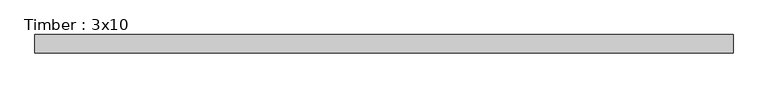
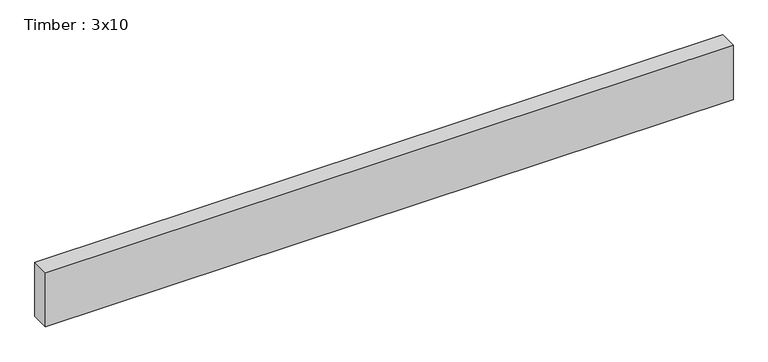
"""IFC4 building model written with IfcOpenShell, lengths in millimetres: beam geometry, Timber : 3x10."""

import ifcopenshell
import ifcopenshell.guid

model = None  # the IFC model being written
_history = None  # IfcOwnerHistory: only IFC2X3 demands one
_inside = {}  # id of a spatial element -> (the spatial element, [elements in it])
_under = {}  # id of a project, library or spatial element -> (it, [spatial elements below it])
_declared = {}  # id of a project -> (the project, [libraries it declares])
_typed = {}  # id of a type object -> (the type object, [elements of that type])
_made_of = {}  # id of a material, layer set ... -> (it, [elements and type objects made of it])


def new_model(schema):
    """Start an empty IFC model of exactly this schema.

    Asked for "IFC4X3", IfcOpenShell would pick the latest addendum, in which some entities
    have other attributes; the version numbers below select the first issue.
    IFC2X3 requires an IfcOwnerHistory on every rooted entity: one is made here for all.
    """
    global model, _history
    if schema == "IFC4X3":
        model = ifcopenshell.file(schema_version=(4, 3, 0, 0))
    else:
        model = ifcopenshell.file(schema=schema)
    _inside.clear()
    _under.clear()
    _declared.clear()
    _typed.clear()
    _made_of.clear()
    _history = None
    if model.schema == "IFC2X3":
        org = make("IfcOrganization", Name="unknown")
        user = make(
            "IfcPersonAndOrganization",
            ThePerson=make("IfcPerson", FamilyName="unknown"),
            TheOrganization=org,
        )
        app = make(
            "IfcApplication",
            ApplicationDeveloper=org,
            Version="unknown",
            ApplicationFullName="unknown",
            ApplicationIdentifier="unknown",
        )
        _history = make(
            "IfcOwnerHistory",
            OwningUser=user,
            OwningApplication=app,
            ChangeAction="ADDED",
            CreationDate=0,
        )
    return model


def make(cls, **values):
    """One entity of the class cls with the attributes given. An attribute that is None is left unset."""
    return model.create_entity(
        cls, **{name: value for name, value in values.items() if value is not None}
    )


def rooted(cls, **values):
    """An entity with a GlobalId (a new one), such as an element, a storey or a relation."""
    return make(cls, GlobalId=ifcopenshell.guid.new(), OwnerHistory=_history, **values)


def si_unit(unit_type, name, prefix=None):
    """IfcSIUnit, for example si_unit("LENGTHUNIT", "METRE", prefix="MILLI")."""
    return make("IfcSIUnit", UnitType=unit_type, Prefix=prefix, Name=name)


def assignment(units):
    """IfcUnitAssignment: the units of a project."""
    return None if units is None else make("IfcUnitAssignment", Units=units)


def point(xyz):
    """IfcCartesianPoint."""
    return None if xyz is None else make("IfcCartesianPoint", Coordinates=xyz)


def direction(xyz):
    """IfcDirection."""
    return None if xyz is None else make("IfcDirection", DirectionRatios=xyz)


def frame(location, z_axis=None, x_axis=None):
    """IfcAxis2Placement3D, a coordinate frame: its origin and axes. An axis left out is left unset."""
    return make(
        "IfcAxis2Placement3D",
        Location=point(location),
        Axis=direction(z_axis),
        RefDirection=direction(x_axis),
    )


def origin():
    """The frame at (0, 0, 0) with its axes left unset."""
    return frame((0.0, 0.0, 0.0))


def place(relative_to, where):
    """IfcLocalPlacement: puts the frame where relative to a parent placement (None: the world)."""
    return make(
        "IfcLocalPlacement", PlacementRelTo=relative_to, RelativePlacement=where
    )


def context(
    kind, dimensions, precision=None, world=None, true_north=None, identifier=None
):
    """IfcGeometricRepresentationContext, for example the 3D "Model" context."""
    return make(
        "IfcGeometricRepresentationContext",
        ContextIdentifier=identifier,
        ContextType=kind,
        CoordinateSpaceDimension=dimensions,
        Precision=precision,
        WorldCoordinateSystem=world,
        TrueNorth=true_north,
    )


def project(units=None, contexts=None):
    """IfcProject with its units and contexts."""
    return rooted(
        "IfcProject",
        Name="project",
        RepresentationContexts=contexts,
        UnitsInContext=assignment(units),
    )


def spatial(cls, under=None, at=None, **own):
    """A site, building, storey or space (cls), placed at a placement, below another one or the project."""
    s = rooted(cls, ObjectPlacement=at, **own)
    if under is not None:
        _under.setdefault(under.id(), (under, []))[1].append(s)
    return s


def polyline(points):
    """IfcPolyline through the points."""
    return make("IfcPolyline", Points=[point(p) for p in points])


def outline(outer, holes=None, kind="AREA"):
    """IfcArbitraryClosedProfileDef: a profile drawn as a closed curve; with holes, ...WithVoids."""
    if holes is None:
        return make("IfcArbitraryClosedProfileDef", ProfileType=kind, OuterCurve=outer)
    return make(
        "IfcArbitraryProfileDefWithVoids",
        ProfileType=kind,
        OuterCurve=outer,
        InnerCurves=holes,
    )


def extrude(swept, where, along, depth):
    """IfcExtrudedAreaSolid: the profile swept, set in the frame where, extruded along a direction by depth."""
    return make(
        "IfcExtrudedAreaSolid",
        SweptArea=swept,
        Position=where,
        ExtrudedDirection=direction(along),
        Depth=depth,
    )


def shape(context_of_items, identifier, shape_type, items):
    """IfcShapeRepresentation: the items that make up one representation, for example the "Body"."""
    return make(
        "IfcShapeRepresentation",
        ContextOfItems=context_of_items,
        RepresentationIdentifier=identifier,
        RepresentationType=shape_type,
        Items=items,
    )


def source(mapping_origin, context_of_items, identifier, shape_type, items):
    """IfcRepresentationMap: a shape defined once, which mapped items show again and again."""
    return make(
        "IfcRepresentationMap",
        MappingOrigin=mapping_origin,
        MappedRepresentation=shape(context_of_items, identifier, shape_type, items),
    )


def transform(
    local_origin,
    x_axis=None,
    y_axis=None,
    z_axis=None,
    scale=None,
    scale2=None,
    scale3=None,
    uniform=True,
):
    """IfcCartesianTransformationOperator3D, or its non-uniform kind. x_axis, y_axis, z_axis: its Axis1, 2, 3."""
    if uniform:
        return make(
            "IfcCartesianTransformationOperator3D",
            Axis1=direction(x_axis),
            Axis2=direction(y_axis),
            LocalOrigin=point(local_origin),
            Scale=scale,
            Axis3=direction(z_axis),
        )
    return make(
        "IfcCartesianTransformationOperator3DnonUniform",
        Axis1=direction(x_axis),
        Axis2=direction(y_axis),
        LocalOrigin=point(local_origin),
        Scale=scale,
        Axis3=direction(z_axis),
        Scale2=scale2,
        Scale3=scale3,
    )


def mapped(mapping_source, mapping_target):
    """IfcMappedItem: shows the shape of a source again, moved by a transform."""
    return make(
        "IfcMappedItem", MappingSource=mapping_source, MappingTarget=mapping_target
    )


def made_of(thing, what):
    """Note that an element or type object is made of a material, layer set ...; save() writes the relation."""
    if what is not None:
        _made_of.setdefault(what.id(), (what, []))[1].append(thing)
    return thing


def element(
    cls,
    number,
    at=None,
    inside=None,
    cuts=None,
    type_object=None,
    material=None,
    context=None,
    identifier="Body",
    shape_type=None,
    held_by="IfcProductDefinitionShape",
    body=None,
    shapes=None,
    **own,
):
    """One element of the class cls, such as IfcWall. Its Tag is "e" and its number.

    at: its placement. inside: the storey or other place that contains it. cuts: it is an
    opening in that element (IfcRelVoidsElement). A single representation is given by context,
    identifier, shape_type and body (its items); several are given by shapes. held_by: the class
    of the entity that holds the representations. save() writes the other relations.
    """
    e = rooted(cls, Tag="e%d" % number, ObjectPlacement=at, **own)
    if body is not None:
        shapes = [shape(context, identifier, shape_type, body)]
    if shapes is not None:
        e.Representation = make(held_by, Representations=shapes)
    if inside is not None:
        _inside.setdefault(inside.id(), (inside, []))[1].append(e)
    if cuts is not None:
        rooted(
            "IfcRelVoidsElement", RelatingBuildingElement=cuts, RelatedOpeningElement=e
        )
    if type_object is not None:
        _typed.setdefault(type_object.id(), (type_object, []))[1].append(e)
    return made_of(e, material)


def aggregate(whole, parts):
    """IfcRelAggregates: a whole, such as a stair, and the parts it consists of."""
    return rooted("IfcRelAggregates", RelatingObject=whole, RelatedObjects=parts)


def save(model, path):
    """Write the relations noted so far, then the file.

    IfcRelAggregates (storeys below a building ...), IfcRelContainedInSpatialStructure (elements
    in a storey), IfcRelDefinesByType, IfcRelAssociatesMaterial and IfcRelDeclares: one each for
    every whole, place, type object, material and project.
    """
    for whole, parts in _under.values():
        aggregate(whole, parts)
    for where, things in _inside.values():
        rooted(
            "IfcRelContainedInSpatialStructure",
            RelatedElements=things,
            RelatingStructure=where,
        )
    for kind, things in _typed.values():
        rooted("IfcRelDefinesByType", RelatedObjects=things, RelatingType=kind)
    for what, things in _made_of.values():
        rooted("IfcRelAssociatesMaterial", RelatedObjects=things, RelatingMaterial=what)
    for by, libraries in _declared.values():
        rooted("IfcRelDeclares", RelatingContext=by, RelatedDefinitions=libraries)
    model.write(path)


def timber_3x10_f201f224(model_context):
    return source(origin(), model_context, "Body", "SweptSolid", [
        extrude(outline(polyline([(1446.1657684, 38.1), (1446.1657684, -38.1), (-1446.1657684, -38.1), (-1446.1657684, 38.1), (1446.1657684, 38.1)])), frame((0.0, 0.0, -120.65), z_axis=(0.0, 0.0, 1.0), x_axis=(1.0, 0.0, 0.0)), (0.0, 0.0, 1.0), 241.3),
    ])


if __name__ == "__main__":
    model = new_model("IFC4")
    model_context = context("Model", 3, world=origin())
    ifc_project = project(units=[si_unit("LENGTHUNIT", "METRE", prefix="MILLI")], contexts=[model_context])
    site = spatial("IfcSite", under=ifc_project)
    building = spatial("IfcBuilding", under=site)
    placement = place(None, origin())
    timber_3x10_shape = timber_3x10_f201f224(model_context)
    element("IfcBeam", 1, ObjectType="Timber : 3x10", at=placement, inside=building, context=model_context, shape_type="MappedRepresentation", body=[
        mapped(timber_3x10_shape, transform((0.0, 0.0, 0.0), x_axis=(1.0, 0.0, 0.0), y_axis=(0.0, 1.0, 0.0), z_axis=(0.0, 0.0, 1.0))),
    ])
    save(model, "model.ifc")

# Revit data of these elements
# Type "Timber : 3x10"
#   Assembly Code = "B10"
#   A = 0.362847 SF
#   Length [instance default] = 5' - 0"
#   b = 0' - 3"
#   d = 0' - 9 1/2"
#   Structural Material [instance default] = Softwood, Lumber
# Element 1 (IfcBeam, "Timber : 3x10")
#   Materials on its faces: "Softwood, Lumber"
# Materials
#   "Softwood, Lumber": class "Wood", colour RGB 144 113 62, transparency 0, Description = "Pinus Echinata", Cost = 0
